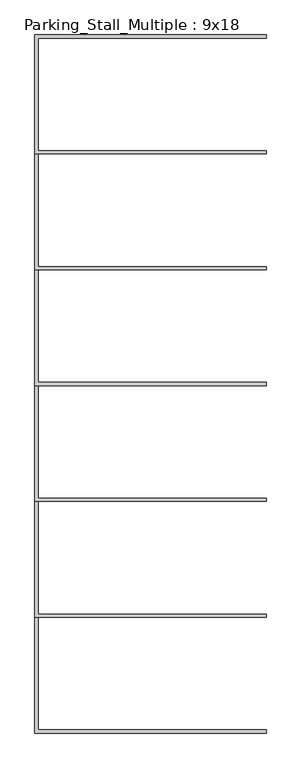
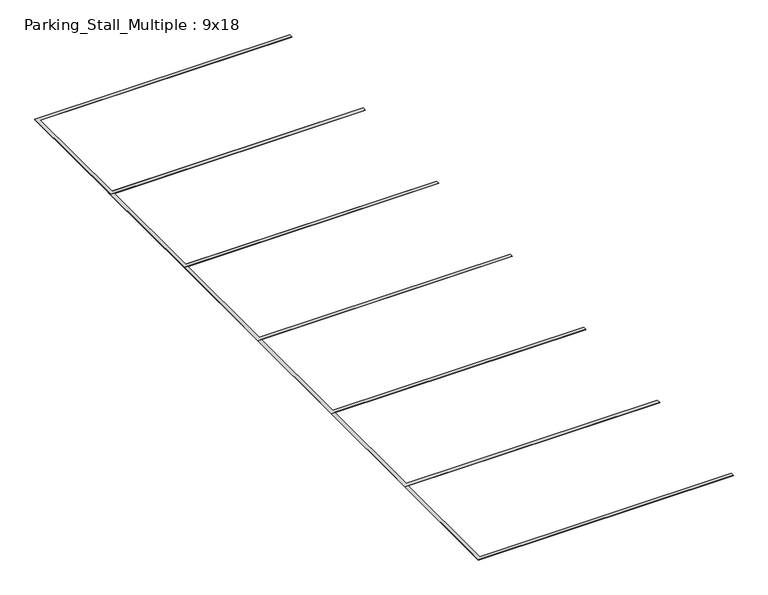
"""IFC4 building model written with IfcOpenShell, lengths in millimetres: proxy geometry, Parking_Stall_Multiple : 9x18."""

from ifc_helpers import new_model, si_unit, origin, origin_with_axes, place, context, project, spatial, polyline, outline, extrude, source, transform, mapped, element, save


def parking_stall_multiple_9x18_96eb0467(model_context):
    return source(origin(), model_context, "Body", "SweptSolid", [
        extrude(outline(polyline([(5486.4, 13716.0), (0.0, 13716.0), (0.0, 16535.4), (5486.4, 16535.4), (5486.4, 16459.2), (76.2, 16459.2), (76.2, 13792.2), (5486.4, 13792.2), (5486.4, 13716.0)])), origin_with_axes(), (0.0, 0.0, 1.0), 6.35),
        extrude(outline(polyline([(5486.4, 10972.8), (0.0, 10972.8), (0.0, 13792.2), (5486.4, 13792.2), (5486.4, 13716.0), (76.2, 13716.0), (76.2, 11049.0), (5486.4, 11049.0), (5486.4, 10972.8)])), origin_with_axes(), (0.0, 0.0, 1.0), 6.35),
        extrude(outline(polyline([(5486.4, 8229.6), (0.0, 8229.6), (0.0, 11049.0), (5486.4, 11049.0), (5486.4, 10972.8), (76.2, 10972.8), (76.2, 8305.8), (5486.4, 8305.8), (5486.4, 8229.6)])), origin_with_axes(), (0.0, 0.0, 1.0), 6.35),
        extrude(outline(polyline([(5486.4, 5486.4), (0.0, 5486.4), (0.0, 8305.8), (5486.4, 8305.8), (5486.4, 8229.6), (76.2, 8229.6), (76.2, 5562.6), (5486.4, 5562.6), (5486.4, 5486.4)])), origin_with_axes(), (0.0, 0.0, 1.0), 6.35),
        extrude(outline(polyline([(5486.4, 2743.2), (0.0, 2743.2), (0.0, 5562.6), (5486.4, 5562.6), (5486.4, 5486.4), (76.2, 5486.4), (76.2, 2819.4), (5486.4, 2819.4), (5486.4, 2743.2)])), origin_with_axes(), (0.0, 0.0, 1.0), 6.35),
        extrude(outline(polyline([(5486.4, 0.0), (0.0, 0.0), (0.0, 2819.4), (5486.4, 2819.4), (5486.4, 2743.2), (76.2, 2743.2), (76.2, 76.2), (5486.4, 76.2), (5486.4, 0.0)])), origin_with_axes(), (0.0, 0.0, 1.0), 6.35),
    ])


if __name__ == "__main__":
    model = new_model("IFC4")
    model_context = context("Model", 3, world=origin())
    ifc_project = project(units=[si_unit("LENGTHUNIT", "METRE", prefix="MILLI")], contexts=[model_context])
    site = spatial("IfcSite", under=ifc_project)
    building = spatial("IfcBuilding", under=site)
    placement = place(None, origin())
    parking_stall_multiple_9x18_shape = parking_stall_multiple_9x18_96eb0467(model_context)
    element("IfcBuildingElementProxy", 1, Name="Parking_Stall_Multiple : 9x18", ObjectType="Parking_Stall_Multiple : 9x18", at=placement, inside=building, context=model_context, shape_type="MappedRepresentation", body=[
        mapped(parking_stall_multiple_9x18_shape, transform((0.0, 0.0, 0.0), x_axis=(1.0, 0.0, 0.0), y_axis=(0.0, 1.0, 0.0), z_axis=(0.0, 0.0, 1.0))),
    ])
    save(model, "model.ifc")

# Revit data of these elements
# Type "Parking_Stall_Multiple : 9x18"
#   Parking_Width_M = 9' - 0"
#   Parking_Run_Length [instance default] = 65' - 0"
#   Parking_Line_Width = 0' - 3"
#   Parking_Length_M = 18' - 0"
#   Single_Parking_Visibility [instance default] = no
#   Parking_ADA_Symbol = no
#   ParkingUnitsArray [instance default] = 7
#   ParkingUnits [instance default] = 7
#   Multiple_Parking_Visibility [instance default] = yes
#   Parking_Line_Material = ADA VAN ACCESSIBLE STALL
# Element 1 (IfcBuildingElementProxy, "Parking_Stall_Multiple : 9x18")
#   Parking_Run_Length = 50' - 7.16009"
#   ParkingUnitsArray = 6
#   ParkingUnits = 6
#   Materials on its faces: "ADA VAN ACCESSIBLE STALL"
# Materials
#   "ADA VAN ACCESSIBLE STALL": class "Paint", colour RGB 255 255 255, transparency 0, Cost = 0
